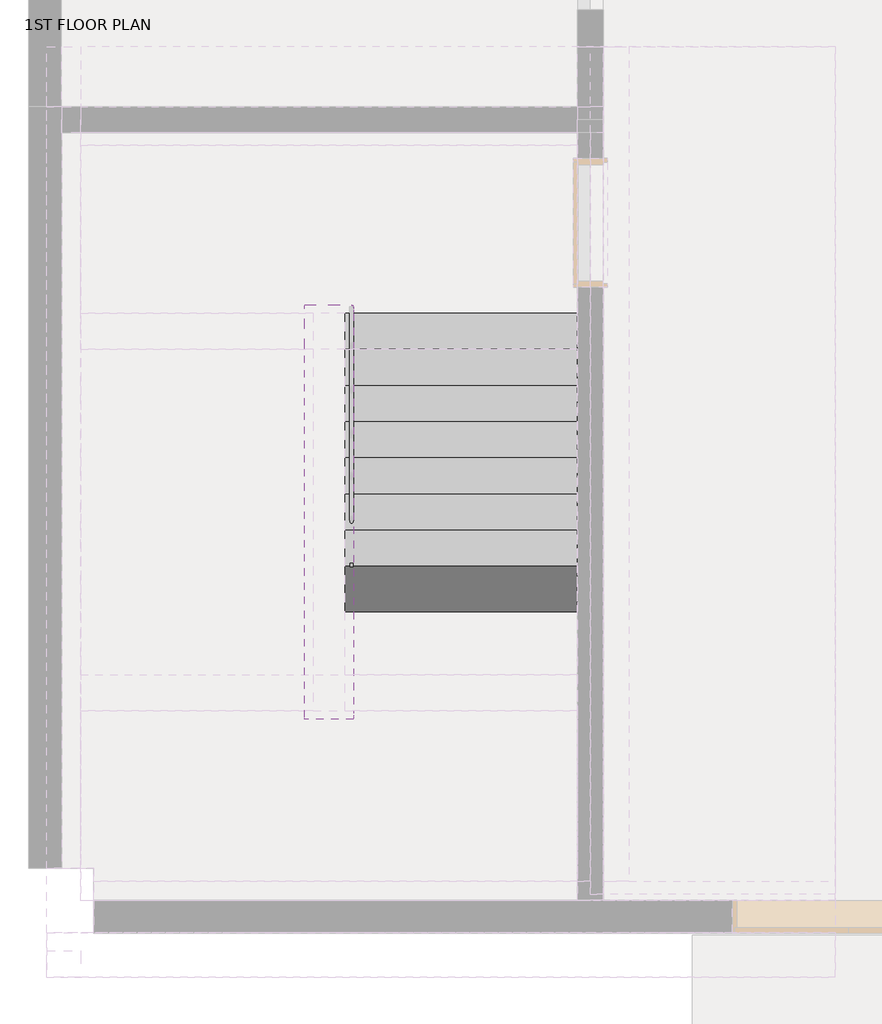
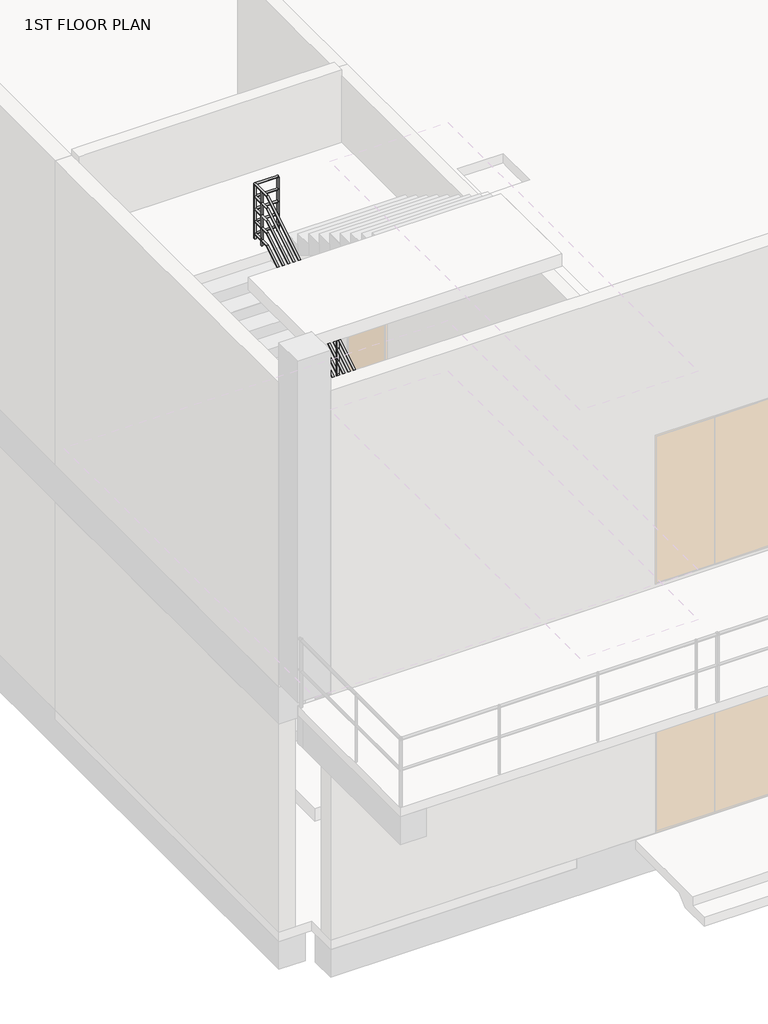
# One storey, part 8 of 9: 1 railing, 1 stair flight.
"""IFC4 building model written with IfcOpenShell, lengths in millimetres."""

from ifc_helpers import new_model, si_unit, frame, origin, place, context, project, spatial, polyline, circle_curve, ellipse_curve, outline, extrude, faceted_brep, element, save
from ifc_brep_helpers import plane_surface, cylinder_surface, advanced_brep

model = new_model("IFC4")

# Units and contexts
model_context = context("Model", 3, world=origin())
ifc_project = project(units=[si_unit("LENGTHUNIT", "METRE", prefix="MILLI")], contexts=[model_context])

# Site, building, storey
site = spatial("IfcSite", under=ifc_project)
building = spatial("IfcBuilding", under=site)
storey = spatial("IfcBuildingStorey", under=building, Name="1ST FLOOR PLAN", Elevation=600.005241)

# Railing
placement = place(None, origin())
element("IfcRailing", 1, ObjectType="900mm 배관", at=placement, inside=storey, context=model_context, shape_type="SolidModel", body=[
    advanced_brep(
    [(2135.0, 25549.5208589, 5485.005241), (2165.0, 25549.5208589, 5485.005241), (2135.0, 25495.2843108, 5485.005241), (2165.0, 25495.2843108, 5485.005241), (2135.0, 22415.2843108, 7375.630241), (2165.0, 22415.2843108, 7375.630241), (2135.0, 22384.5208589, 7375.630241), (2165.0, 22354.5208589, 7375.630241), (1800.0, 22384.5208589, 7375.630241), (1800.0, 22354.5208589, 7375.630241)],
    [
        (0, 1, circle_curve(frame((2150.0, 25549.5208589, 5485.005241), z_axis=(0.0, 1.0, 0.0), x_axis=(1.0, 0.0, 0.0)), 15.0)),
        (1, 0, circle_curve(frame((2150.0, 25549.5208589, 5485.005241), z_axis=(0.0, 1.0, 0.0), x_axis=(1.0, 0.0, 0.0)), 15.0)),
        (0, 2),
        (2, 3, ellipse_curve(frame((2150.0, 25495.2843108, 5485.005241), z_axis=(0.0, 0.9623527489128249, -0.2718035810285242), x_axis=(0.0, 0.2718035810285241, 0.9623527489128249)), 15.5868002, 15.0)),
        (3, 1),
        (3, 2, ellipse_curve(frame((2150.0, 25495.2843108, 5485.005241), z_axis=(0.0, 0.9623527489128249, -0.2718035810285242), x_axis=(0.0, 0.2718035810285241, 0.9623527489128249)), 15.5868002, 15.0)),
        (2, 4),
        (4, 5, ellipse_curve(frame((2150.0, 22415.2843108, 7375.630241), z_axis=(0.0, 0.9623527489128249, -0.27180358102852414), x_axis=(0.0, -0.2718035810285245, -0.9623527489128249)), 15.5868002, 15.0)),
        (5, 3),
        (5, 4, ellipse_curve(frame((2150.0, 22415.2843108, 7375.630241), z_axis=(0.0, 0.9623527489128249, -0.27180358102852414), x_axis=(0.0, -0.2718035810285245, -0.9623527489128249)), 15.5868002, 15.0)),
        (4, 6),
        (6, 7, ellipse_curve(frame((2150.0, 22369.5208589, 7375.630241), z_axis=(0.7071067811865475, 0.7071067811865475, 0.0), x_axis=(-0.7071067811865474, 0.7071067811865476, 0.0)), 21.2132034, 15.0)),
        (7, 5),
        (7, 6, ellipse_curve(frame((2150.0, 22369.5208589, 7375.630241), z_axis=(0.7071067811865475, 0.7071067811865475, 0.0), x_axis=(-0.7071067811865474, 0.7071067811865476, 0.0)), 21.2132034, 15.0)),
        (8, 9, ellipse_curve(frame((1800.0, 22369.5208589, 7375.630241), z_axis=(-0.7071067811865476, 0.0, 0.7071067811865476), x_axis=(0.7071067811865475, 0.0, 0.7071067811865476)), 21.2132034, 15.0)),
        (9, 8, ellipse_curve(frame((1800.0, 22369.5208589, 7375.630241), z_axis=(-0.7071067811865476, 0.0, 0.7071067811865476), x_axis=(0.7071067811865475, 0.0, 0.7071067811865476)), 21.2132034, 15.0)),
        (6, 8),
        (9, 7),
    ],
    [
        plane_surface(frame((2150.0, 25549.5208589, 5500.005241), z_axis=(0.0, 1.0, 0.0), x_axis=(0.0, 0.0, -1.0))),
        cylinder_surface(frame((2150.0, 25549.5208589, 5485.005241), z_axis=(0.0, 1.0, 0.0), x_axis=(1.0, 0.0, 0.0)), 15.0),
        cylinder_surface(frame((2150.0, 25491.6737312, 5487.2215566), z_axis=(0.0, 0.852245626680141, -0.5231418467343), x_axis=(1.0, 0.0, 0.0)), 15.0),
        cylinder_surface(frame((2150.0, 22419.5208589, 7375.630241), z_axis=(0.0, 1.0, 0.0), x_axis=(1.0, 0.0, 0.0)), 15.0),
        plane_surface(frame((1815.0, 22369.5208589, 7390.630241), z_axis=(-0.7071067811865476, 0.0, 0.7071067811865476), x_axis=(0.7071067811865476, 0.0, 0.7071067811865476))),
        cylinder_surface(frame((2150.0, 22369.5208589, 7375.630241), z_axis=(1.0, 0.0, 0.0), x_axis=(0.0, -1.0, 0.0)), 15.0),
    ],
    [
        (0, [[1, 2]]),
        (1, [[-1, 3, 4, 5]]),
        (1, [[-2, -5, 6, -3]]),
        (2, [[-4, 7, 8, 9]]),
        (2, [[-6, -9, 10, -7]]),
        (3, [[-8, 11, 12, 13]]),
        (3, [[-10, -13, 14, -11]]),
        (4, [[15, 16]]),
        (5, [[-12, 17, -16, 18]]),
        (5, [[-14, -18, -15, -17]]),
    ],
),
    advanced_brep(
    [(1800.0, 22384.5208589, 7375.630241), (1800.0, 22354.5208589, 7375.630241), (1800.0, 22384.5208589, 7505.8197466), (1800.0, 22354.5208589, 7522.6056874)],
    [
        (0, 1, ellipse_curve(frame((1800.0, 22369.5208589, 7375.630241), z_axis=(0.7071067811865476, 0.0, -0.7071067811865476), x_axis=(-0.7071067811865476, 0.0, -0.7071067811865474)), 21.2132034, 15.0)),
        (1, 0, ellipse_curve(frame((1800.0, 22369.5208589, 7375.630241), z_axis=(0.7071067811865476, 0.0, -0.7071067811865476), x_axis=(-0.7071067811865476, 0.0, -0.7071067811865474)), 21.2132034, 15.0)),
        (2, 3, ellipse_curve(frame((1800.0, 22369.5208589, 7514.212717), z_axis=(0.0, 0.48829199935371653, 0.8726803099458301), x_axis=(0.0, 0.8726803099458301, -0.4882919993537164)), 17.1884249, 15.0)),
        (3, 2, ellipse_curve(frame((1800.0, 22369.5208589, 7514.212717), z_axis=(0.0, 0.48829199935371653, 0.8726803099458301), x_axis=(0.0, 0.8726803099458301, -0.4882919993537164)), 17.1884249, 15.0)),
        (0, 2),
        (3, 1),
    ],
    [
        plane_surface(frame((1800.0, 22369.5208589, 7375.630241), z_axis=(0.7071067811865476, 0.0, -0.7071067811865476), x_axis=(0.7071067811865476, 0.0, 0.7071067811865476))),
        plane_surface(frame((1800.0, 22369.5208589, 7514.212717), z_axis=(0.0, 0.48829199935371653, 0.8726803099458301), x_axis=(1.0, 0.0, 0.0))),
        cylinder_surface(frame((1800.0, 22369.5208589, 7375.630241), z_axis=(0.0, 0.0, -1.0), x_axis=(0.0, -1.0, 0.0)), 15.0),
    ],
    [
        (0, [[1, 2]]),
        (1, [[3, 4]]),
        (2, [[-1, 5, -4, 6]]),
        (2, [[-2, -6, -3, -5]]),
    ],
),
    advanced_brep(
    [(1815.0, 22369.5208589, 7514.212717), (1785.0, 22369.5208589, 7514.212717), (1815.0, 25223.757407, 9266.255241), (1785.0, 25223.757407, 9266.255241), (1815.0, 25534.5208589, 9266.255241), (1785.0, 25564.5208589, 9266.255241), (2150.0, 25534.5208589, 9266.255241), (2150.0, 25564.5208589, 9266.255241)],
    [
        (0, 1, ellipse_curve(frame((1800.0, 22369.5208589, 7514.212717), z_axis=(0.0, -0.48829199935371653, -0.8726803099458301), x_axis=(0.0, -0.8726803099458302, 0.48829199935371653)), 17.1884249, 15.0)),
        (1, 0, ellipse_curve(frame((1800.0, 22369.5208589, 7514.212717), z_axis=(0.0, -0.48829199935371653, -0.8726803099458301), x_axis=(0.0, -0.8726803099458302, 0.48829199935371653)), 17.1884249, 15.0)),
        (0, 2),
        (2, 3, ellipse_curve(frame((1800.0, 25223.757407, 9266.255241), z_axis=(0.0, -0.9623527489128247, -0.27180358102852437), x_axis=(0.0, 0.2718035810285242, -0.9623527489128249)), 15.5868002, 15.0)),
        (3, 1),
        (3, 2, ellipse_curve(frame((1800.0, 25223.757407, 9266.255241), z_axis=(0.0, -0.9623527489128247, -0.27180358102852437), x_axis=(0.0, 0.2718035810285242, -0.9623527489128249)), 15.5868002, 15.0)),
        (2, 4),
        (4, 5, ellipse_curve(frame((1800.0, 25549.5208589, 9266.255241), z_axis=(-0.7071067811865475, -0.7071067811865475, 0.0), x_axis=(0.7071067811865474, -0.7071067811865476, 0.0)), 21.2132034, 15.0)),
        (5, 3),
        (5, 4, ellipse_curve(frame((1800.0, 25549.5208589, 9266.255241), z_axis=(-0.7071067811865475, -0.7071067811865475, 0.0), x_axis=(0.7071067811865474, -0.7071067811865476, 0.0)), 21.2132034, 15.0)),
        (6, 7, circle_curve(frame((2150.0, 25549.5208589, 9266.255241), z_axis=(1.0, 0.0, 0.0), x_axis=(0.0, 1.0, 0.0)), 15.0)),
        (7, 6, circle_curve(frame((2150.0, 25549.5208589, 9266.255241), z_axis=(1.0, 0.0, 0.0), x_axis=(0.0, 1.0, 0.0)), 15.0)),
        (4, 6),
        (7, 5),
    ],
    [
        plane_surface(frame((1800.0, 22354.5208589, 7522.6056874), z_axis=(0.0, -0.48829199935371653, -0.8726803099458301), x_axis=(1.0, 0.0, 0.0))),
        cylinder_surface(frame((1800.0, 22362.3679866, 7509.822003), z_axis=(0.0, -0.8522456266801408, -0.5231418467343004), x_axis=(-1.0, 0.0, 0.0)), 15.0),
        cylinder_surface(frame((1800.0, 25219.5208589, 9266.255241), z_axis=(0.0, -1.0, 0.0), x_axis=(-1.0, 0.0, 0.0)), 15.0),
        plane_surface(frame((2150.0, 25549.5208589, 9281.255241), z_axis=(1.0, 0.0, 0.0), x_axis=(0.0, 1.0, 0.0))),
        cylinder_surface(frame((1800.0, 25549.5208589, 9266.255241), z_axis=(-1.0, 0.0, 0.0), x_axis=(0.0, 1.0, 0.0)), 15.0),
    ],
    [
        (0, [[1, 2]]),
        (1, [[-1, 3, 4, 5]]),
        (1, [[-2, -5, 6, -3]]),
        (2, [[-4, 7, 8, 9]]),
        (2, [[-6, -9, 10, -7]]),
        (3, [[11, 12]]),
        (4, [[-8, 13, -12, 14]]),
        (4, [[-10, -14, -11, -13]]),
    ],
),
    advanced_brep(
    [(2165.0, 25549.5208589, 5285.005241), (2135.0, 25549.5208589, 5285.005241), (2165.0, 25495.2843108, 5285.005241), (2135.0, 25495.2843108, 5285.005241), (2165.0, 22415.2843108, 7175.630241), (2135.0, 22415.2843108, 7175.630241), (2165.0, 22384.5208589, 7175.630241), (2135.0, 22384.5208589, 7175.630241)],
    [
        (0, 1, circle_curve(frame((2150.0, 25549.5208589, 5285.005241), z_axis=(0.0, 1.0, 0.0), x_axis=(-1.0, 0.0, 0.0)), 15.0)),
        (1, 0, circle_curve(frame((2150.0, 25549.5208589, 5285.005241), z_axis=(0.0, 1.0, 0.0), x_axis=(-1.0, 0.0, 0.0)), 15.0)),
        (0, 2),
        (2, 3, ellipse_curve(frame((2150.0, 25495.2843108, 5285.005241), z_axis=(0.0, 0.9623527489128249, -0.2718035810285242), x_axis=(0.0, 0.2718035810285241, 0.9623527489128249)), 15.5868002, 15.0)),
        (3, 1),
        (3, 2, ellipse_curve(frame((2150.0, 25495.2843108, 5285.005241), z_axis=(0.0, 0.9623527489128249, -0.2718035810285242), x_axis=(0.0, 0.2718035810285241, 0.9623527489128249)), 15.5868002, 15.0)),
        (2, 4),
        (4, 5, ellipse_curve(frame((2150.0, 22415.2843108, 7175.630241), z_axis=(0.0, 0.9623527489128249, -0.27180358102852414), x_axis=(0.0, -0.2718035810285245, -0.9623527489128249)), 15.5868002, 15.0)),
        (5, 3),
        (5, 4, ellipse_curve(frame((2150.0, 22415.2843108, 7175.630241), z_axis=(0.0, 0.9623527489128249, -0.27180358102852414), x_axis=(0.0, -0.2718035810285245, -0.9623527489128249)), 15.5868002, 15.0)),
        (6, 7, circle_curve(frame((2150.0, 22384.5208589, 7175.630241), z_axis=(0.0, -1.0, 0.0), x_axis=(-1.0, 0.0, 0.0)), 15.0)),
        (7, 6, circle_curve(frame((2150.0, 22384.5208589, 7175.630241), z_axis=(0.0, -1.0, 0.0), x_axis=(-1.0, 0.0, 0.0)), 15.0)),
        (4, 6),
        (7, 5),
    ],
    [
        plane_surface(frame((2150.0, 25549.5208589, 5300.005241), z_axis=(0.0, 1.0, 0.0), x_axis=(0.0, 0.0, -1.0))),
        cylinder_surface(frame((2150.0, 25549.5208589, 5285.005241), z_axis=(0.0, 1.0, 0.0), x_axis=(-1.0, 0.0, 0.0)), 15.0),
        cylinder_surface(frame((2150.0, 25491.6737312, 5287.2215566), z_axis=(0.0, 0.852245626680141, -0.5231418467343), x_axis=(-1.0, 0.0, 0.0)), 15.0),
        plane_surface(frame((2150.0, 22384.5208589, 7190.630241), z_axis=(0.0, -1.0, 0.0), x_axis=(0.0, 0.0, -1.0))),
        cylinder_surface(frame((2150.0, 22419.5208589, 7175.630241), z_axis=(0.0, 1.0, 0.0), x_axis=(-1.0, 0.0, 0.0)), 15.0),
    ],
    [
        (0, [[1, 2]]),
        (1, [[-1, 3, 4, 5]]),
        (1, [[-2, -5, 6, -3]]),
        (2, [[-4, 7, 8, 9]]),
        (2, [[-6, -9, 10, -7]]),
        (3, [[11, 12]]),
        (4, [[-8, 13, -12, 14]]),
        (4, [[-10, -14, -11, -13]]),
    ],
),
    advanced_brep(
    [(2165.0, 22354.5208589, 7175.630241), (2165.0, 22384.5208589, 7175.630241), (1815.0, 22354.5208589, 7175.630241), (1815.0, 22384.5208589, 7175.630241)],
    [
        (0, 1, circle_curve(frame((2165.0, 22369.5208589, 7175.630241), z_axis=(1.0, 0.0, 0.0), x_axis=(0.0, 1.0, 0.0)), 15.0)),
        (1, 0, circle_curve(frame((2165.0, 22369.5208589, 7175.630241), z_axis=(1.0, 0.0, 0.0), x_axis=(0.0, 1.0, 0.0)), 15.0)),
        (2, 3, circle_curve(frame((1815.0, 22369.5208589, 7175.630241), z_axis=(-1.0, 0.0, 0.0), x_axis=(0.0, 1.0, 0.0)), 15.0)),
        (3, 2, circle_curve(frame((1815.0, 22369.5208589, 7175.630241), z_axis=(-1.0, 0.0, 0.0), x_axis=(0.0, 1.0, 0.0)), 15.0)),
        (0, 2),
        (3, 1),
    ],
    [
        plane_surface(frame((2165.0, 22369.5208589, 7190.630241), z_axis=(1.0, 0.0, 0.0), x_axis=(0.0, -1.0, 0.0))),
        plane_surface(frame((1815.0, 22369.5208589, 7190.630241), z_axis=(-1.0, 0.0, 0.0), x_axis=(0.0, -1.0, 0.0))),
        cylinder_surface(frame((2165.0, 22369.5208589, 7175.630241), z_axis=(1.0, 0.0, 0.0), x_axis=(0.0, 1.0, 0.0)), 15.0),
    ],
    [
        (0, [[1, 2]]),
        (1, [[3, 4]]),
        (2, [[-1, 5, -4, 6]]),
        (2, [[-2, -6, -3, -5]]),
    ],
),
    advanced_brep(
    [(1785.0, 22354.5208589, 7305.0051277), (1815.0, 22354.5208589, 7305.0051277), (1785.0, 25223.757407, 9066.255241), (1815.0, 25223.757407, 9066.255241), (1785.0, 25534.5208589, 9066.255241), (1815.0, 25534.5208589, 9066.255241)],
    [
        (0, 1, ellipse_curve(frame((1800.0, 22354.5208589, 7305.0051277), z_axis=(0.0, -1.0, 0.0), x_axis=(0.0, 0.0, -1.0)), 17.6005597, 15.0)),
        (1, 0, ellipse_curve(frame((1800.0, 22354.5208589, 7305.0051277), z_axis=(0.0, -1.0, 0.0), x_axis=(0.0, 0.0, -1.0)), 17.6005597, 15.0)),
        (0, 2),
        (2, 3, ellipse_curve(frame((1800.0, 25223.757407, 9066.255241), z_axis=(0.0, -0.9623527489128247, -0.27180358102852437), x_axis=(0.0, 0.2718035810285242, -0.9623527489128249)), 15.5868002, 15.0)),
        (3, 1),
        (3, 2, ellipse_curve(frame((1800.0, 25223.757407, 9066.255241), z_axis=(0.0, -0.9623527489128247, -0.27180358102852437), x_axis=(0.0, 0.2718035810285242, -0.9623527489128249)), 15.5868002, 15.0)),
        (4, 5, circle_curve(frame((1800.0, 25534.5208589, 9066.255241), z_axis=(0.0, 1.0, 0.0), x_axis=(1.0, 0.0, 0.0)), 15.0)),
        (5, 4, circle_curve(frame((1800.0, 25534.5208589, 9066.255241), z_axis=(0.0, 1.0, 0.0), x_axis=(1.0, 0.0, 0.0)), 15.0)),
        (2, 4),
        (5, 3),
    ],
    [
        plane_surface(frame((1800.0, 22354.5208589, 7322.6056874), z_axis=(0.0, -1.0, 0.0), x_axis=(0.0, 0.0, 1.0))),
        cylinder_surface(frame((1800.0, 22362.3679866, 7309.822003), z_axis=(0.0, -0.8522456266801408, -0.5231418467343004), x_axis=(1.0, 0.0, 0.0)), 15.0),
        plane_surface(frame((1800.0, 25534.5208589, 9081.255241), z_axis=(0.0, 1.0, 0.0), x_axis=(0.0, 0.0, 1.0))),
        cylinder_surface(frame((1800.0, 25219.5208589, 9066.255241), z_axis=(0.0, -1.0, 0.0), x_axis=(1.0, 0.0, 0.0)), 15.0),
    ],
    [
        (0, [[1, 2]]),
        (1, [[-1, 3, 4, 5]]),
        (1, [[-2, -5, 6, -3]]),
        (2, [[7, 8]]),
        (3, [[-4, 9, -8, 10]]),
        (3, [[-6, -10, -7, -9]]),
    ],
),
    advanced_brep(
    [(1785.0, 25564.5208589, 9066.255241), (1785.0, 25534.5208589, 9066.255241), (2150.0, 25564.5208589, 9066.255241), (2150.0, 25534.5208589, 9066.255241)],
    [
        (0, 1, circle_curve(frame((1785.0, 25549.5208589, 9066.255241), z_axis=(-1.0, 0.0, 0.0), x_axis=(0.0, -1.0, 0.0)), 15.0)),
        (1, 0, circle_curve(frame((1785.0, 25549.5208589, 9066.255241), z_axis=(-1.0, 0.0, 0.0), x_axis=(0.0, -1.0, 0.0)), 15.0)),
        (2, 3, circle_curve(frame((2150.0, 25549.5208589, 9066.255241), z_axis=(1.0, 0.0, 0.0), x_axis=(0.0, -1.0, 0.0)), 15.0)),
        (3, 2, circle_curve(frame((2150.0, 25549.5208589, 9066.255241), z_axis=(1.0, 0.0, 0.0), x_axis=(0.0, -1.0, 0.0)), 15.0)),
        (0, 2),
        (3, 1),
    ],
    [
        plane_surface(frame((1785.0, 25549.5208589, 9081.255241), z_axis=(-1.0, 0.0, 0.0), x_axis=(0.0, 1.0, 0.0))),
        plane_surface(frame((2150.0, 25549.5208589, 9081.255241), z_axis=(1.0, 0.0, 0.0), x_axis=(0.0, 1.0, 0.0))),
        cylinder_surface(frame((1785.0, 25549.5208589, 9066.255241), z_axis=(-1.0, 0.0, 0.0), x_axis=(0.0, -1.0, 0.0)), 15.0),
    ],
    [
        (0, [[1, 2]]),
        (1, [[3, 4]]),
        (2, [[-1, 5, -4, 6]]),
        (2, [[-2, -6, -3, -5]]),
    ],
),
    advanced_brep(
    [(2165.0, 25549.5208589, 5085.005241), (2135.0, 25549.5208589, 5085.005241), (2165.0, 25495.2843108, 5085.005241), (2135.0, 25495.2843108, 5085.005241), (2165.0, 22415.2843108, 6975.630241), (2135.0, 22415.2843108, 6975.630241), (2165.0, 22384.5208589, 6975.630241), (2135.0, 22384.5208589, 6975.630241)],
    [
        (0, 1, circle_curve(frame((2150.0, 25549.5208589, 5085.005241), z_axis=(0.0, 1.0, 0.0), x_axis=(-1.0, 0.0, 0.0)), 15.0)),
        (1, 0, circle_curve(frame((2150.0, 25549.5208589, 5085.005241), z_axis=(0.0, 1.0, 0.0), x_axis=(-1.0, 0.0, 0.0)), 15.0)),
        (0, 2),
        (2, 3, ellipse_curve(frame((2150.0, 25495.2843108, 5085.005241), z_axis=(0.0, 0.9623527489128249, -0.2718035810285242), x_axis=(0.0, 0.2718035810285241, 0.9623527489128249)), 15.5868002, 15.0)),
        (3, 1),
        (3, 2, ellipse_curve(frame((2150.0, 25495.2843108, 5085.005241), z_axis=(0.0, 0.9623527489128249, -0.2718035810285242), x_axis=(0.0, 0.2718035810285241, 0.9623527489128249)), 15.5868002, 15.0)),
        (2, 4),
        (4, 5, ellipse_curve(frame((2150.0, 22415.2843108, 6975.630241), z_axis=(0.0, 0.9623527489128249, -0.27180358102852414), x_axis=(0.0, -0.2718035810285245, -0.9623527489128249)), 15.5868002, 15.0)),
        (5, 3),
        (5, 4, ellipse_curve(frame((2150.0, 22415.2843108, 6975.630241), z_axis=(0.0, 0.9623527489128249, -0.27180358102852414), x_axis=(0.0, -0.2718035810285245, -0.9623527489128249)), 15.5868002, 15.0)),
        (6, 7, circle_curve(frame((2150.0, 22384.5208589, 6975.630241), z_axis=(0.0, -1.0, 0.0), x_axis=(-1.0, 0.0, 0.0)), 15.0)),
        (7, 6, circle_curve(frame((2150.0, 22384.5208589, 6975.630241), z_axis=(0.0, -1.0, 0.0), x_axis=(-1.0, 0.0, 0.0)), 15.0)),
        (4, 6),
        (7, 5),
    ],
    [
        plane_surface(frame((2150.0, 25549.5208589, 5100.005241), z_axis=(0.0, 1.0, 0.0), x_axis=(0.0, 0.0, -1.0))),
        cylinder_surface(frame((2150.0, 25549.5208589, 5085.005241), z_axis=(0.0, 1.0, 0.0), x_axis=(-1.0, 0.0, 0.0)), 15.0),
        cylinder_surface(frame((2150.0, 25491.6737312, 5087.2215566), z_axis=(0.0, 0.852245626680141, -0.5231418467343), x_axis=(-1.0, 0.0, 0.0)), 15.0),
        plane_surface(frame((2150.0, 22384.5208589, 6990.630241), z_axis=(0.0, -1.0, 0.0), x_axis=(0.0, 0.0, -1.0))),
        cylinder_surface(frame((2150.0, 22419.5208589, 6975.630241), z_axis=(0.0, 1.0, 0.0), x_axis=(-1.0, 0.0, 0.0)), 15.0),
    ],
    [
        (0, [[1, 2]]),
        (1, [[-1, 3, 4, 5]]),
        (1, [[-2, -5, 6, -3]]),
        (2, [[-4, 7, 8, 9]]),
        (2, [[-6, -9, 10, -7]]),
        (3, [[11, 12]]),
        (4, [[-8, 13, -12, 14]]),
        (4, [[-10, -14, -11, -13]]),
    ],
),
    advanced_brep(
    [(2165.0, 22354.5208589, 6975.630241), (2165.0, 22384.5208589, 6975.630241), (1815.0, 22354.5208589, 6975.630241), (1815.0, 22384.5208589, 6975.630241)],
    [
        (0, 1, circle_curve(frame((2165.0, 22369.5208589, 6975.630241), z_axis=(1.0, 0.0, 0.0), x_axis=(0.0, 1.0, 0.0)), 15.0)),
        (1, 0, circle_curve(frame((2165.0, 22369.5208589, 6975.630241), z_axis=(1.0, 0.0, 0.0), x_axis=(0.0, 1.0, 0.0)), 15.0)),
        (2, 3, circle_curve(frame((1815.0, 22369.5208589, 6975.630241), z_axis=(-1.0, 0.0, 0.0), x_axis=(0.0, 1.0, 0.0)), 15.0)),
        (3, 2, circle_curve(frame((1815.0, 22369.5208589, 6975.630241), z_axis=(-1.0, 0.0, 0.0), x_axis=(0.0, 1.0, 0.0)), 15.0)),
        (0, 2),
        (3, 1),
    ],
    [
        plane_surface(frame((2165.0, 22369.5208589, 6990.630241), z_axis=(1.0, 0.0, 0.0), x_axis=(0.0, -1.0, 0.0))),
        plane_surface(frame((1815.0, 22369.5208589, 6990.630241), z_axis=(-1.0, 0.0, 0.0), x_axis=(0.0, -1.0, 0.0))),
        cylinder_surface(frame((2165.0, 22369.5208589, 6975.630241), z_axis=(1.0, 0.0, 0.0), x_axis=(0.0, 1.0, 0.0)), 15.0),
    ],
    [
        (0, [[1, 2]]),
        (1, [[3, 4]]),
        (2, [[-1, 5, -4, 6]]),
        (2, [[-2, -6, -3, -5]]),
    ],
),
    advanced_brep(
    [(1785.0, 22354.5208589, 7105.0051277), (1815.0, 22354.5208589, 7105.0051277), (1785.0, 25223.757407, 8866.255241), (1815.0, 25223.757407, 8866.255241), (1785.0, 25534.5208589, 8866.255241), (1815.0, 25534.5208589, 8866.255241)],
    [
        (0, 1, ellipse_curve(frame((1800.0, 22354.5208589, 7105.0051277), z_axis=(0.0, -1.0, 0.0), x_axis=(0.0, 0.0, -1.0)), 17.6005597, 15.0)),
        (1, 0, ellipse_curve(frame((1800.0, 22354.5208589, 7105.0051277), z_axis=(0.0, -1.0, 0.0), x_axis=(0.0, 0.0, -1.0)), 17.6005597, 15.0)),
        (0, 2),
        (2, 3, ellipse_curve(frame((1800.0, 25223.757407, 8866.255241), z_axis=(0.0, -0.9623527489128247, -0.27180358102852437), x_axis=(0.0, 0.2718035810285242, -0.9623527489128249)), 15.5868002, 15.0)),
        (3, 1),
        (3, 2, ellipse_curve(frame((1800.0, 25223.757407, 8866.255241), z_axis=(0.0, -0.9623527489128247, -0.27180358102852437), x_axis=(0.0, 0.2718035810285242, -0.9623527489128249)), 15.5868002, 15.0)),
        (4, 5, circle_curve(frame((1800.0, 25534.5208589, 8866.255241), z_axis=(0.0, 1.0, 0.0), x_axis=(1.0, 0.0, 0.0)), 15.0)),
        (5, 4, circle_curve(frame((1800.0, 25534.5208589, 8866.255241), z_axis=(0.0, 1.0, 0.0), x_axis=(1.0, 0.0, 0.0)), 15.0)),
        (2, 4),
        (5, 3),
    ],
    [
        plane_surface(frame((1800.0, 22354.5208589, 7122.6056874), z_axis=(0.0, -1.0, 0.0), x_axis=(0.0, 0.0, 1.0))),
        cylinder_surface(frame((1800.0, 22362.3679866, 7109.822003), z_axis=(0.0, -0.8522456266801408, -0.5231418467343004), x_axis=(1.0, 0.0, 0.0)), 15.0),
        plane_surface(frame((1800.0, 25534.5208589, 8881.255241), z_axis=(0.0, 1.0, 0.0), x_axis=(0.0, 0.0, 1.0))),
        cylinder_surface(frame((1800.0, 25219.5208589, 8866.255241), z_axis=(0.0, -1.0, 0.0), x_axis=(1.0, 0.0, 0.0)), 15.0),
    ],
    [
        (0, [[1, 2]]),
        (1, [[-1, 3, 4, 5]]),
        (1, [[-2, -5, 6, -3]]),
        (2, [[7, 8]]),
        (3, [[-4, 9, -8, 10]]),
        (3, [[-6, -10, -7, -9]]),
    ],
),
    advanced_brep(
    [(1785.0, 25564.5208589, 8866.255241), (1785.0, 25534.5208589, 8866.255241), (2150.0, 25564.5208589, 8866.255241), (2150.0, 25534.5208589, 8866.255241)],
    [
        (0, 1, circle_curve(frame((1785.0, 25549.5208589, 8866.255241), z_axis=(-1.0, 0.0, 0.0), x_axis=(0.0, -1.0, 0.0)), 15.0)),
        (1, 0, circle_curve(frame((1785.0, 25549.5208589, 8866.255241), z_axis=(-1.0, 0.0, 0.0), x_axis=(0.0, -1.0, 0.0)), 15.0)),
        (2, 3, circle_curve(frame((2150.0, 25549.5208589, 8866.255241), z_axis=(1.0, 0.0, 0.0), x_axis=(0.0, -1.0, 0.0)), 15.0)),
        (3, 2, circle_curve(frame((2150.0, 25549.5208589, 8866.255241), z_axis=(1.0, 0.0, 0.0), x_axis=(0.0, -1.0, 0.0)), 15.0)),
        (0, 2),
        (3, 1),
    ],
    [
        plane_surface(frame((1785.0, 25549.5208589, 8881.255241), z_axis=(-1.0, 0.0, 0.0), x_axis=(0.0, 1.0, 0.0))),
        plane_surface(frame((2150.0, 25549.5208589, 8881.255241), z_axis=(1.0, 0.0, 0.0), x_axis=(0.0, 1.0, 0.0))),
        cylinder_surface(frame((1785.0, 25549.5208589, 8866.255241), z_axis=(-1.0, 0.0, 0.0), x_axis=(0.0, -1.0, 0.0)), 15.0),
    ],
    [
        (0, [[1, 2]]),
        (1, [[3, 4]]),
        (2, [[-1, 5, -4, 6]]),
        (2, [[-2, -6, -3, -5]]),
    ],
),
    advanced_brep(
    [(2165.0, 25549.5208589, 4885.005241), (2135.0, 25549.5208589, 4885.005241), (2165.0, 25495.2843108, 4885.005241), (2135.0, 25495.2843108, 4885.005241), (2165.0, 22415.2843108, 6775.630241), (2135.0, 22415.2843108, 6775.630241), (2165.0, 22384.5208589, 6775.630241), (2135.0, 22384.5208589, 6775.630241)],
    [
        (0, 1, circle_curve(frame((2150.0, 25549.5208589, 4885.005241), z_axis=(0.0, 1.0, 0.0), x_axis=(-1.0, 0.0, 0.0)), 15.0)),
        (1, 0, circle_curve(frame((2150.0, 25549.5208589, 4885.005241), z_axis=(0.0, 1.0, 0.0), x_axis=(-1.0, 0.0, 0.0)), 15.0)),
        (0, 2),
        (2, 3, ellipse_curve(frame((2150.0, 25495.2843108, 4885.005241), z_axis=(0.0, 0.9623527489128249, -0.2718035810285242), x_axis=(0.0, 0.2718035810285241, 0.9623527489128249)), 15.5868002, 15.0)),
        (3, 1),
        (3, 2, ellipse_curve(frame((2150.0, 25495.2843108, 4885.005241), z_axis=(0.0, 0.9623527489128249, -0.2718035810285242), x_axis=(0.0, 0.2718035810285241, 0.9623527489128249)), 15.5868002, 15.0)),
        (2, 4),
        (4, 5, ellipse_curve(frame((2150.0, 22415.2843108, 6775.630241), z_axis=(0.0, 0.9623527489128249, -0.27180358102852414), x_axis=(0.0, -0.2718035810285245, -0.9623527489128249)), 15.5868002, 15.0)),
        (5, 3),
        (5, 4, ellipse_curve(frame((2150.0, 22415.2843108, 6775.630241), z_axis=(0.0, 0.9623527489128249, -0.27180358102852414), x_axis=(0.0, -0.2718035810285245, -0.9623527489128249)), 15.5868002, 15.0)),
        (6, 7, circle_curve(frame((2150.0, 22384.5208589, 6775.630241), z_axis=(0.0, -1.0, 0.0), x_axis=(-1.0, 0.0, 0.0)), 15.0)),
        (7, 6, circle_curve(frame((2150.0, 22384.5208589, 6775.630241), z_axis=(0.0, -1.0, 0.0), x_axis=(-1.0, 0.0, 0.0)), 15.0)),
        (4, 6),
        (7, 5),
    ],
    [
        plane_surface(frame((2150.0, 25549.5208589, 4900.005241), z_axis=(0.0, 1.0, 0.0), x_axis=(0.0, 0.0, -1.0))),
        cylinder_surface(frame((2150.0, 25549.5208589, 4885.005241), z_axis=(0.0, 1.0, 0.0), x_axis=(-1.0, 0.0, 0.0)), 15.0),
        cylinder_surface(frame((2150.0, 25491.6737312, 4887.2215566), z_axis=(0.0, 0.852245626680141, -0.5231418467343), x_axis=(-1.0, 0.0, 0.0)), 15.0),
        plane_surface(frame((2150.0, 22384.5208589, 6790.630241), z_axis=(0.0, -1.0, 0.0), x_axis=(0.0, 0.0, -1.0))),
        cylinder_surface(frame((2150.0, 22419.5208589, 6775.630241), z_axis=(0.0, 1.0, 0.0), x_axis=(-1.0, 0.0, 0.0)), 15.0),
    ],
    [
        (0, [[1, 2]]),
        (1, [[-1, 3, 4, 5]]),
        (1, [[-2, -5, 6, -3]]),
        (2, [[-4, 7, 8, 9]]),
        (2, [[-6, -9, 10, -7]]),
        (3, [[11, 12]]),
        (4, [[-8, 13, -12, 14]]),
        (4, [[-10, -14, -11, -13]]),
    ],
),
    advanced_brep(
    [(2165.0, 22354.5208589, 6775.630241), (2165.0, 22384.5208589, 6775.630241), (1815.0, 22354.5208589, 6775.630241), (1815.0, 22384.5208589, 6775.630241)],
    [
        (0, 1, circle_curve(frame((2165.0, 22369.5208589, 6775.630241), z_axis=(1.0, 0.0, 0.0), x_axis=(0.0, 1.0, 0.0)), 15.0)),
        (1, 0, circle_curve(frame((2165.0, 22369.5208589, 6775.630241), z_axis=(1.0, 0.0, 0.0), x_axis=(0.0, 1.0, 0.0)), 15.0)),
        (2, 3, circle_curve(frame((1815.0, 22369.5208589, 6775.630241), z_axis=(-1.0, 0.0, 0.0), x_axis=(0.0, 1.0, 0.0)), 15.0)),
        (3, 2, circle_curve(frame((1815.0, 22369.5208589, 6775.630241), z_axis=(-1.0, 0.0, 0.0), x_axis=(0.0, 1.0, 0.0)), 15.0)),
        (0, 2),
        (3, 1),
    ],
    [
        plane_surface(frame((2165.0, 22369.5208589, 6790.630241), z_axis=(1.0, 0.0, 0.0), x_axis=(0.0, -1.0, 0.0))),
        plane_surface(frame((1815.0, 22369.5208589, 6790.630241), z_axis=(-1.0, 0.0, 0.0), x_axis=(0.0, -1.0, 0.0))),
        cylinder_surface(frame((2165.0, 22369.5208589, 6775.630241), z_axis=(1.0, 0.0, 0.0), x_axis=(0.0, 1.0, 0.0)), 15.0),
    ],
    [
        (0, [[1, 2]]),
        (1, [[3, 4]]),
        (2, [[-1, 5, -4, 6]]),
        (2, [[-2, -6, -3, -5]]),
    ],
),
    advanced_brep(
    [(1785.0, 22354.5208589, 6905.0051277), (1815.0, 22354.5208589, 6905.0051277), (1785.0, 25223.757407, 8666.255241), (1815.0, 25223.757407, 8666.255241), (1785.0, 25534.5208589, 8666.255241), (1815.0, 25534.5208589, 8666.255241)],
    [
        (0, 1, ellipse_curve(frame((1800.0, 22354.5208589, 6905.0051277), z_axis=(0.0, -1.0, 0.0), x_axis=(0.0, 0.0, -1.0)), 17.6005597, 15.0)),
        (1, 0, ellipse_curve(frame((1800.0, 22354.5208589, 6905.0051277), z_axis=(0.0, -1.0, 0.0), x_axis=(0.0, 0.0, -1.0)), 17.6005597, 15.0)),
        (0, 2),
        (2, 3, ellipse_curve(frame((1800.0, 25223.757407, 8666.255241), z_axis=(0.0, -0.9623527489128247, -0.27180358102852437), x_axis=(0.0, 0.2718035810285242, -0.9623527489128249)), 15.5868002, 15.0)),
        (3, 1),
        (3, 2, ellipse_curve(frame((1800.0, 25223.757407, 8666.255241), z_axis=(0.0, -0.9623527489128247, -0.27180358102852437), x_axis=(0.0, 0.2718035810285242, -0.9623527489128249)), 15.5868002, 15.0)),
        (4, 5, circle_curve(frame((1800.0, 25534.5208589, 8666.255241), z_axis=(0.0, 1.0, 0.0), x_axis=(1.0, 0.0, 0.0)), 15.0)),
        (5, 4, circle_curve(frame((1800.0, 25534.5208589, 8666.255241), z_axis=(0.0, 1.0, 0.0), x_axis=(1.0, 0.0, 0.0)), 15.0)),
        (2, 4),
        (5, 3),
    ],
    [
        plane_surface(frame((1800.0, 22354.5208589, 6922.6056874), z_axis=(0.0, -1.0, 0.0), x_axis=(0.0, 0.0, 1.0))),
        cylinder_surface(frame((1800.0, 22362.3679866, 6909.822003), z_axis=(0.0, -0.8522456266801408, -0.5231418467343004), x_axis=(1.0, 0.0, 0.0)), 15.0),
        plane_surface(frame((1800.0, 25534.5208589, 8681.255241), z_axis=(0.0, 1.0, 0.0), x_axis=(0.0, 0.0, 1.0))),
        cylinder_surface(frame((1800.0, 25219.5208589, 8666.255241), z_axis=(0.0, -1.0, 0.0), x_axis=(1.0, 0.0, 0.0)), 15.0),
    ],
    [
        (0, [[1, 2]]),
        (1, [[-1, 3, 4, 5]]),
        (1, [[-2, -5, 6, -3]]),
        (2, [[7, 8]]),
        (3, [[-4, 9, -8, 10]]),
        (3, [[-6, -10, -7, -9]]),
    ],
),
    advanced_brep(
    [(1785.0, 25564.5208589, 8666.255241), (1785.0, 25534.5208589, 8666.255241), (2150.0, 25564.5208589, 8666.255241), (2150.0, 25534.5208589, 8666.255241)],
    [
        (0, 1, circle_curve(frame((1785.0, 25549.5208589, 8666.255241), z_axis=(-1.0, 0.0, 0.0), x_axis=(0.0, -1.0, 0.0)), 15.0)),
        (1, 0, circle_curve(frame((1785.0, 25549.5208589, 8666.255241), z_axis=(-1.0, 0.0, 0.0), x_axis=(0.0, -1.0, 0.0)), 15.0)),
        (2, 3, circle_curve(frame((2150.0, 25549.5208589, 8666.255241), z_axis=(1.0, 0.0, 0.0), x_axis=(0.0, -1.0, 0.0)), 15.0)),
        (3, 2, circle_curve(frame((2150.0, 25549.5208589, 8666.255241), z_axis=(1.0, 0.0, 0.0), x_axis=(0.0, -1.0, 0.0)), 15.0)),
        (0, 2),
        (3, 1),
    ],
    [
        plane_surface(frame((1785.0, 25549.5208589, 8681.255241), z_axis=(-1.0, 0.0, 0.0), x_axis=(0.0, 1.0, 0.0))),
        plane_surface(frame((2150.0, 25549.5208589, 8681.255241), z_axis=(1.0, 0.0, 0.0), x_axis=(0.0, 1.0, 0.0))),
        cylinder_surface(frame((1785.0, 25549.5208589, 8666.255241), z_axis=(-1.0, 0.0, 0.0), x_axis=(0.0, -1.0, 0.0)), 15.0),
    ],
    [
        (0, [[1, 2]]),
        (1, [[3, 4]]),
        (2, [[-1, 5, -4, 6]]),
        (2, [[-2, -6, -3, -5]]),
    ],
),
    advanced_brep(
    [(2165.0, 25549.5208589, 4685.005241), (2135.0, 25549.5208589, 4685.005241), (2165.0, 25495.2843108, 4685.005241), (2135.0, 25495.2843108, 4685.005241), (2165.0, 22415.2843108, 6575.630241), (2135.0, 22415.2843108, 6575.630241), (2165.0, 22384.5208589, 6575.630241), (2135.0, 22384.5208589, 6575.630241)],
    [
        (0, 1, circle_curve(frame((2150.0, 25549.5208589, 4685.005241), z_axis=(0.0, 1.0, 0.0), x_axis=(-1.0, 0.0, 0.0)), 15.0)),
        (1, 0, circle_curve(frame((2150.0, 25549.5208589, 4685.005241), z_axis=(0.0, 1.0, 0.0), x_axis=(-1.0, 0.0, 0.0)), 15.0)),
        (0, 2),
        (2, 3, ellipse_curve(frame((2150.0, 25495.2843108, 4685.005241), z_axis=(0.0, 0.9623527489128249, -0.2718035810285242), x_axis=(0.0, 0.2718035810285241, 0.9623527489128249)), 15.5868002, 15.0)),
        (3, 1),
        (3, 2, ellipse_curve(frame((2150.0, 25495.2843108, 4685.005241), z_axis=(0.0, 0.9623527489128249, -0.2718035810285242), x_axis=(0.0, 0.2718035810285241, 0.9623527489128249)), 15.5868002, 15.0)),
        (2, 4),
        (4, 5, ellipse_curve(frame((2150.0, 22415.2843108, 6575.630241), z_axis=(0.0, 0.9623527489128249, -0.27180358102852414), x_axis=(0.0, -0.2718035810285245, -0.9623527489128249)), 15.5868002, 15.0)),
        (5, 3),
        (5, 4, ellipse_curve(frame((2150.0, 22415.2843108, 6575.630241), z_axis=(0.0, 0.9623527489128249, -0.27180358102852414), x_axis=(0.0, -0.2718035810285245, -0.9623527489128249)), 15.5868002, 15.0)),
        (6, 7, circle_curve(frame((2150.0, 22384.5208589, 6575.630241), z_axis=(0.0, -1.0, 0.0), x_axis=(-1.0, 0.0, 0.0)), 15.0)),
        (7, 6, circle_curve(frame((2150.0, 22384.5208589, 6575.630241), z_axis=(0.0, -1.0, 0.0), x_axis=(-1.0, 0.0, 0.0)), 15.0)),
        (4, 6),
        (7, 5),
    ],
    [
        plane_surface(frame((2150.0, 25549.5208589, 4700.005241), z_axis=(0.0, 1.0, 0.0), x_axis=(0.0, 0.0, -1.0))),
        cylinder_surface(frame((2150.0, 25549.5208589, 4685.005241), z_axis=(0.0, 1.0, 0.0), x_axis=(-1.0, 0.0, 0.0)), 15.0),
        cylinder_surface(frame((2150.0, 25491.6737312, 4687.2215566), z_axis=(0.0, 0.852245626680141, -0.5231418467343), x_axis=(-1.0, 0.0, 0.0)), 15.0),
        plane_surface(frame((2150.0, 22384.5208589, 6590.630241), z_axis=(0.0, -1.0, 0.0), x_axis=(0.0, 0.0, -1.0))),
        cylinder_surface(frame((2150.0, 22419.5208589, 6575.630241), z_axis=(0.0, 1.0, 0.0), x_axis=(-1.0, 0.0, 0.0)), 15.0),
    ],
    [
        (0, [[1, 2]]),
        (1, [[-1, 3, 4, 5]]),
        (1, [[-2, -5, 6, -3]]),
        (2, [[-4, 7, 8, 9]]),
        (2, [[-6, -9, 10, -7]]),
        (3, [[11, 12]]),
        (4, [[-8, 13, -12, 14]]),
        (4, [[-10, -14, -11, -13]]),
    ],
),
    advanced_brep(
    [(2165.0, 22354.5208589, 6575.630241), (2165.0, 22384.5208589, 6575.630241), (1815.0, 22354.5208589, 6575.630241), (1815.0, 22384.5208589, 6575.630241)],
    [
        (0, 1, circle_curve(frame((2165.0, 22369.5208589, 6575.630241), z_axis=(1.0, 0.0, 0.0), x_axis=(0.0, 1.0, 0.0)), 15.0)),
        (1, 0, circle_curve(frame((2165.0, 22369.5208589, 6575.630241), z_axis=(1.0, 0.0, 0.0), x_axis=(0.0, 1.0, 0.0)), 15.0)),
        (2, 3, circle_curve(frame((1815.0, 22369.5208589, 6575.630241), z_axis=(-1.0, 0.0, 0.0), x_axis=(0.0, 1.0, 0.0)), 15.0)),
        (3, 2, circle_curve(frame((1815.0, 22369.5208589, 6575.630241), z_axis=(-1.0, 0.0, 0.0), x_axis=(0.0, 1.0, 0.0)), 15.0)),
        (0, 2),
        (3, 1),
    ],
    [
        plane_surface(frame((2165.0, 22369.5208589, 6590.630241), z_axis=(1.0, 0.0, 0.0), x_axis=(0.0, -1.0, 0.0))),
        plane_surface(frame((1815.0, 22369.5208589, 6590.630241), z_axis=(-1.0, 0.0, 0.0), x_axis=(0.0, -1.0, 0.0))),
        cylinder_surface(frame((2165.0, 22369.5208589, 6575.630241), z_axis=(1.0, 0.0, 0.0), x_axis=(0.0, 1.0, 0.0)), 15.0),
    ],
    [
        (0, [[1, 2]]),
        (1, [[3, 4]]),
        (2, [[-1, 5, -4, 6]]),
        (2, [[-2, -6, -3, -5]]),
    ],
),
    advanced_brep(
    [(1785.0, 22354.5208589, 6705.0051277), (1815.0, 22354.5208589, 6705.0051277), (1785.0, 25223.757407, 8466.255241), (1815.0, 25223.757407, 8466.255241), (1785.0, 25534.5208589, 8466.255241), (1815.0, 25534.5208589, 8466.255241)],
    [
        (0, 1, ellipse_curve(frame((1800.0, 22354.5208589, 6705.0051277), z_axis=(0.0, -1.0, 0.0), x_axis=(0.0, 0.0, -1.0)), 17.6005597, 15.0)),
        (1, 0, ellipse_curve(frame((1800.0, 22354.5208589, 6705.0051277), z_axis=(0.0, -1.0, 0.0), x_axis=(0.0, 0.0, -1.0)), 17.6005597, 15.0)),
        (0, 2),
        (2, 3, ellipse_curve(frame((1800.0, 25223.757407, 8466.255241), z_axis=(0.0, -0.9623527489128247, -0.27180358102852437), x_axis=(0.0, 0.2718035810285242, -0.9623527489128249)), 15.5868002, 15.0)),
        (3, 1),
        (3, 2, ellipse_curve(frame((1800.0, 25223.757407, 8466.255241), z_axis=(0.0, -0.9623527489128247, -0.27180358102852437), x_axis=(0.0, 0.2718035810285242, -0.9623527489128249)), 15.5868002, 15.0)),
        (4, 5, circle_curve(frame((1800.0, 25534.5208589, 8466.255241), z_axis=(0.0, 1.0, 0.0), x_axis=(1.0, 0.0, 0.0)), 15.0)),
        (5, 4, circle_curve(frame((1800.0, 25534.5208589, 8466.255241), z_axis=(0.0, 1.0, 0.0), x_axis=(1.0, 0.0, 0.0)), 15.0)),
        (2, 4),
        (5, 3),
    ],
    [
        plane_surface(frame((1800.0, 22354.5208589, 6722.6056874), z_axis=(0.0, -1.0, 0.0), x_axis=(0.0, 0.0, 1.0))),
        cylinder_surface(frame((1800.0, 22362.3679866, 6709.822003), z_axis=(0.0, -0.8522456266801408, -0.5231418467343004), x_axis=(1.0, 0.0, 0.0)), 15.0),
        plane_surface(frame((1800.0, 25534.5208589, 8481.255241), z_axis=(0.0, 1.0, 0.0), x_axis=(0.0, 0.0, 1.0))),
        cylinder_surface(frame((1800.0, 25219.5208589, 8466.255241), z_axis=(0.0, -1.0, 0.0), x_axis=(1.0, 0.0, 0.0)), 15.0),
    ],
    [
        (0, [[1, 2]]),
        (1, [[-1, 3, 4, 5]]),
        (1, [[-2, -5, 6, -3]]),
        (2, [[7, 8]]),
        (3, [[-4, 9, -8, 10]]),
        (3, [[-6, -10, -7, -9]]),
    ],
),
    advanced_brep(
    [(1785.0, 25564.5208589, 8466.255241), (1785.0, 25534.5208589, 8466.255241), (2150.0, 25564.5208589, 8466.255241), (2150.0, 25534.5208589, 8466.255241)],
    [
        (0, 1, circle_curve(frame((1785.0, 25549.5208589, 8466.255241), z_axis=(-1.0, 0.0, 0.0), x_axis=(0.0, -1.0, 0.0)), 15.0)),
        (1, 0, circle_curve(frame((1785.0, 25549.5208589, 8466.255241), z_axis=(-1.0, 0.0, 0.0), x_axis=(0.0, -1.0, 0.0)), 15.0)),
        (2, 3, circle_curve(frame((2150.0, 25549.5208589, 8466.255241), z_axis=(1.0, 0.0, 0.0), x_axis=(0.0, -1.0, 0.0)), 15.0)),
        (3, 2, circle_curve(frame((2150.0, 25549.5208589, 8466.255241), z_axis=(1.0, 0.0, 0.0), x_axis=(0.0, -1.0, 0.0)), 15.0)),
        (0, 2),
        (3, 1),
    ],
    [
        plane_surface(frame((1785.0, 25549.5208589, 8481.255241), z_axis=(-1.0, 0.0, 0.0), x_axis=(0.0, 1.0, 0.0))),
        plane_surface(frame((2150.0, 25549.5208589, 8481.255241), z_axis=(1.0, 0.0, 0.0), x_axis=(0.0, 1.0, 0.0))),
        cylinder_surface(frame((1785.0, 25549.5208589, 8466.255241), z_axis=(-1.0, 0.0, 0.0), x_axis=(0.0, -1.0, 0.0)), 15.0),
    ],
    [
        (0, [[1, 2]]),
        (1, [[3, 4]]),
        (2, [[-1, 5, -4, 6]]),
        (2, [[-2, -6, -3, -5]]),
    ],
),
    extrude(outline(polyline([(1812.5, 25357.0208589), (1787.5, 25357.0208589), (1787.5, 25382.0208589), (1812.5, 25382.0208589), (1812.5, 25357.0208589)])), frame((0.0, 0.0, 8381.255241), z_axis=(0.0, 0.0, 1.0), x_axis=(1.0, 0.0, 0.0)), (0.0, 0.0, 1.0), 870.0),
    extrude(outline(polyline([(24357.0208589, 8716.6177377), (24382.0208589, 8731.9637199), (24382.0208589, 7693.755241), (24357.0208589, 7693.755241), (24357.0208589, 8716.6177377)])), frame((1787.5, 0.0, 0.0), z_axis=(1.0, 0.0, 0.0), x_axis=(0.0, 1.0, 0.0)), (0.0, 0.0, 1.0), 25.0),
    extrude(outline(polyline([(23357.0208589, 8102.778452), (23382.0208589, 8118.1244341), (23382.0208589, 7178.130241), (23357.0208589, 7178.130241), (23357.0208589, 8102.778452)])), frame((1787.5, 0.0, 0.0), z_axis=(1.0, 0.0, 0.0), x_axis=(0.0, 1.0, 0.0)), (0.0, 0.0, 1.0), 25.0),
    extrude(outline(polyline([(22537.0208589, 7283.3030056), (22562.0208589, 7267.9570234), (22562.0208589, 6318.755241), (22537.0208589, 6318.755241), (22537.0208589, 7283.3030056)])), frame((2137.5, 0.0, 0.0), z_axis=(1.0, 0.0, 0.0), x_axis=(0.0, 1.0, 0.0)), (0.0, 0.0, 1.0), 25.0),
    extrude(outline(polyline([(23537.0208589, 6669.4637199), (23562.0208589, 6654.1177377), (23562.0208589, 5631.255241), (23537.0208589, 5631.255241), (23537.0208589, 6669.4637199)])), frame((2137.5, 0.0, 0.0), z_axis=(1.0, 0.0, 0.0), x_axis=(0.0, 1.0, 0.0)), (0.0, 0.0, 1.0), 25.0),
    extrude(outline(polyline([(24537.0208589, 6055.6244341), (24562.0208589, 6040.278452), (24562.0208589, 5115.630241), (24537.0208589, 5115.630241), (24537.0208589, 6055.6244341)])), frame((2137.5, 0.0, 0.0), z_axis=(1.0, 0.0, 0.0), x_axis=(0.0, 1.0, 0.0)), (0.0, 0.0, 1.0), 25.0),
    extrude(outline(polyline([(2137.5, 25537.0208589), (2137.5, 25562.0208589), (2162.5, 25562.0208589), (2162.5, 25537.0208589), (2137.5, 25537.0208589)])), frame((0.0, 0.0, 8381.255241), z_axis=(0.0, 0.0, 1.0), x_axis=(1.0, 0.0, 0.0)), (0.0, 0.0, 1.0), 870.0),
    extrude(outline(polyline([(1812.5, 25537.0208589), (1787.5, 25537.0208589), (1787.5, 25562.0208589), (1812.5, 25562.0208589), (1812.5, 25537.0208589)])), frame((0.0, 0.0, 8381.255241), z_axis=(0.0, 0.0, 1.0), x_axis=(1.0, 0.0, 0.0)), (0.0, 0.0, 1.0), 870.0),
    extrude(outline(polyline([(1812.5, 22382.0208589), (1812.5, 22357.0208589), (1787.5, 22357.0208589), (1787.5, 22382.0208589), (1812.5, 22382.0208589)])), frame((0.0, 0.0, 6490.630241), z_axis=(0.0, 0.0, 1.0), x_axis=(1.0, 0.0, 0.0)), (0.0, 0.0, 1.0), 870.0),
    extrude(outline(polyline([(2137.5, 22382.0208589), (2162.5, 22382.0208589), (2162.5, 22357.0208589), (2137.5, 22357.0208589), (2137.5, 22382.0208589)])), frame((0.0, 0.0, 6490.630241), z_axis=(0.0, 0.0, 1.0), x_axis=(1.0, 0.0, 0.0)), (0.0, 0.0, 1.0), 870.0),
])

# Stair flight
element("IfcStairFlight", 2, ObjectType="1mm 디딤판", at=placement, inside=storey, context=model_context, shape_type="SolidModel", body=[
    faceted_brep([(3900.0, 25219.5208589, 765.8781576), (3900.0, 25499.5208589, 765.8781576), (2100.0, 25499.5208589, 765.8781576), (2100.0, 25219.5208589, 765.8781576), (3900.0, 25219.5208589, 600.005241), (3900.0, 25499.5208589, 600.005241), (2100.0, 25499.5208589, 600.005241), (2100.0, 25219.5208589, 600.005241), (3900.0, 24939.5208589, 932.5448243), (3900.0, 25219.5208589, 932.5448243), (2100.0, 25219.5208589, 932.5448243), (2100.0, 24939.5208589, 932.5448243), (3900.0, 24939.5208589, 757.9826899), (3900.0, 25204.9229731, 600.005241), (2100.0, 25204.9229731, 600.005241), (2100.0, 24939.5208589, 757.9826899), (3900.0, 24659.5208589, 1099.211491), (3900.0, 24939.5208589, 1099.211491), (2100.0, 24939.5208589, 1099.211491), (2100.0, 24659.5208589, 1099.211491), (3900.0, 24659.5208589, 924.6493565), (2100.0, 24659.5208589, 924.6493565), (3900.0, 24379.5208589, 1265.8781576), (3900.0, 24659.5208589, 1265.8781576), (2100.0, 24659.5208589, 1265.8781576), (2100.0, 24379.5208589, 1265.8781576), (3900.0, 24379.5208589, 1091.3160232), (2100.0, 24379.5208589, 1091.3160232), (3900.0, 24099.5208589, 1432.5448243), (3900.0, 24379.5208589, 1432.5448243), (2100.0, 24379.5208589, 1432.5448243), (2100.0, 24099.5208589, 1432.5448243), (3900.0, 24099.5208589, 1257.9826899), (2100.0, 24099.5208589, 1257.9826899), (3900.0, 23819.5208589, 1599.211491), (3900.0, 24099.5208589, 1599.211491), (2100.0, 24099.5208589, 1599.211491), (2100.0, 23819.5208589, 1599.211491), (3900.0, 23819.5208589, 1424.6493565), (2100.0, 23819.5208589, 1424.6493565), (3900.0, 23539.5208589, 1765.8781576), (3900.0, 23819.5208589, 1765.8781576), (2100.0, 23819.5208589, 1765.8781576), (2100.0, 23539.5208589, 1765.8781576), (3900.0, 23539.5208589, 1591.3160232), (2100.0, 23539.5208589, 1591.3160232), (3900.0, 23259.5208589, 1932.5448243), (3900.0, 23539.5208589, 1932.5448243), (2100.0, 23539.5208589, 1932.5448243), (2100.0, 23259.5208589, 1932.5448243), (3900.0, 23259.5208589, 1757.9826899), (2100.0, 23259.5208589, 1757.9826899), (3900.0, 22979.5208589, 2099.211491), (3900.0, 23259.5208589, 2099.211491), (2100.0, 23259.5208589, 2099.211491), (2100.0, 22979.5208589, 2099.211491), (3900.0, 22979.5208589, 1924.6493565), (2100.0, 22979.5208589, 1924.6493565), (3900.0, 22699.5208589, 2265.8781576), (3900.0, 22979.5208589, 2265.8781576), (2100.0, 22979.5208589, 2265.8781576), (2100.0, 22699.5208589, 2265.8781576), (3900.0, 22699.5208589, 2091.3160232), (2100.0, 22699.5208589, 2091.3160232), (3900.0, 22419.5208589, 2432.5448243), (3900.0, 22699.5208589, 2432.5448243), (2100.0, 22699.5208589, 2432.5448243), (2100.0, 22419.5208589, 2432.5448243), (3900.0, 22419.5208589, 2257.9826899), (2100.0, 22419.5208589, 2257.9826899), (2100.0, 22419.5208589, 2399.211491)], [[[0, 1, 2, 3]], [[1, 0, 4, 5]], [[2, 1, 5, 6]], [[3, 2, 6, 7]], [[8, 9, 10, 11]], [[4, 0, 9, 8, 12, 13]], [[0, 3, 10, 9]], [[3, 7, 14, 15, 11, 10]], [[16, 17, 18, 19]], [[17, 16, 20, 12, 8]], [[8, 11, 18, 17]], [[19, 18, 11, 15, 21]], [[22, 23, 24, 25]], [[23, 22, 26, 20, 16]], [[16, 19, 24, 23]], [[25, 24, 19, 21, 27]], [[28, 29, 30, 31]], [[29, 28, 32, 26, 22]], [[22, 25, 30, 29]], [[31, 30, 25, 27, 33]], [[34, 35, 36, 37]], [[35, 34, 38, 32, 28]], [[28, 31, 36, 35]], [[37, 36, 31, 33, 39]], [[40, 41, 42, 43]], [[41, 40, 44, 38, 34]], [[34, 37, 42, 41]], [[43, 42, 37, 39, 45]], [[46, 47, 48, 49]], [[47, 46, 50, 44, 40]], [[40, 43, 48, 47]], [[49, 48, 43, 45, 51]], [[52, 53, 54, 55]], [[53, 52, 56, 50, 46]], [[46, 49, 54, 53]], [[55, 54, 49, 51, 57]], [[58, 59, 60, 61]], [[59, 58, 62, 56, 52]], [[52, 55, 60, 59]], [[61, 60, 55, 57, 63]], [[64, 65, 66, 67]], [[65, 64, 68, 62, 58]], [[58, 61, 66, 65]], [[67, 66, 61, 63, 69, 70]], [[64, 67, 70, 69, 68]], [[5, 4, 13, 14, 7, 6]], [[14, 13, 12, 20, 26, 32, 38, 44, 50, 56, 62, 68, 69, 63, 57, 51, 45, 39, 33, 27, 21, 15]]]),
    extrude(outline(polyline([(3900.0, 25219.5208589), (2100.0, 25219.5208589), (2100.0, 25499.5208589), (3900.0, 25499.5208589), (3900.0, 25219.5208589)])), frame((0.0, 0.0, 765.8781576), z_axis=(0.0, 0.0, 1.0), x_axis=(1.0, 0.0, 0.0)), (0.0, 0.0, 1.0), 0.79375),
    extrude(outline(polyline([(3900.0, 24939.5208589), (2100.0, 24939.5208589), (2100.0, 25219.5208589), (3900.0, 25219.5208589), (3900.0, 24939.5208589)])), frame((0.0, 0.0, 932.5448243), z_axis=(0.0, 0.0, 1.0), x_axis=(1.0, 0.0, 0.0)), (0.0, 0.0, 1.0), 0.79375),
    extrude(outline(polyline([(3900.0, 24659.5208589), (2100.0, 24659.5208589), (2100.0, 24939.5208589), (3900.0, 24939.5208589), (3900.0, 24659.5208589)])), frame((0.0, 0.0, 1099.211491), z_axis=(0.0, 0.0, 1.0), x_axis=(1.0, 0.0, 0.0)), (0.0, 0.0, 1.0), 0.79375),
    extrude(outline(polyline([(3900.0, 24379.5208589), (2100.0, 24379.5208589), (2100.0, 24659.5208589), (3900.0, 24659.5208589), (3900.0, 24379.5208589)])), frame((0.0, 0.0, 1265.8781576), z_axis=(0.0, 0.0, 1.0), x_axis=(1.0, 0.0, 0.0)), (0.0, 0.0, 1.0), 0.79375),
    extrude(outline(polyline([(3900.0, 24099.5208589), (2100.0, 24099.5208589), (2100.0, 24379.5208589), (3900.0, 24379.5208589), (3900.0, 24099.5208589)])), frame((0.0, 0.0, 1432.5448243), z_axis=(0.0, 0.0, 1.0), x_axis=(1.0, 0.0, 0.0)), (0.0, 0.0, 1.0), 0.79375),
    extrude(outline(polyline([(3900.0, 23819.5208589), (2100.0, 23819.5208589), (2100.0, 24099.5208589), (3900.0, 24099.5208589), (3900.0, 23819.5208589)])), frame((0.0, 0.0, 1599.211491), z_axis=(0.0, 0.0, 1.0), x_axis=(1.0, 0.0, 0.0)), (0.0, 0.0, 1.0), 0.79375),
    extrude(outline(polyline([(3900.0, 23539.5208589), (2100.0, 23539.5208589), (2100.0, 23819.5208589), (3900.0, 23819.5208589), (3900.0, 23539.5208589)])), frame((0.0, 0.0, 1765.8781576), z_axis=(0.0, 0.0, 1.0), x_axis=(1.0, 0.0, 0.0)), (0.0, 0.0, 1.0), 0.79375),
    extrude(outline(polyline([(3900.0, 23259.5208589), (2100.0, 23259.5208589), (2100.0, 23539.5208589), (3900.0, 23539.5208589), (3900.0, 23259.5208589)])), frame((0.0, 0.0, 1932.5448243), z_axis=(0.0, 0.0, 1.0), x_axis=(1.0, 0.0, 0.0)), (0.0, 0.0, 1.0), 0.79375),
    extrude(outline(polyline([(3900.0, 22979.5208589), (2100.0, 22979.5208589), (2100.0, 23259.5208589), (3900.0, 23259.5208589), (3900.0, 22979.5208589)])), frame((0.0, 0.0, 2099.211491), z_axis=(0.0, 0.0, 1.0), x_axis=(1.0, 0.0, 0.0)), (0.0, 0.0, 1.0), 0.79375),
    extrude(outline(polyline([(3900.0, 22699.5208589), (2100.0, 22699.5208589), (2100.0, 22979.5208589), (3900.0, 22979.5208589), (3900.0, 22699.5208589)])), frame((0.0, 0.0, 2265.8781576), z_axis=(0.0, 0.0, 1.0), x_axis=(1.0, 0.0, 0.0)), (0.0, 0.0, 1.0), 0.79375),
    extrude(outline(polyline([(3900.0, 22419.5208589), (2100.0, 22419.5208589), (2100.0, 22699.5208589), (3900.0, 22699.5208589), (3900.0, 22419.5208589)])), frame((0.0, 0.0, 2432.5448243), z_axis=(0.0, 0.0, 1.0), x_axis=(1.0, 0.0, 0.0)), (0.0, 0.0, 1.0), 0.79375),
])

save(model, "model.ifc")

# Revit data of these elements
# Type "900mm 배관"
#   built-in parameter 1008612 = 0.019685 (stored number, unit not read)
#   built-in parameter 1008611 = 0.0984252 (stored number, unit not read)
#   built-in parameter 1008609 = 3.28084 (stored number, unit not read)
#   built-in parameter 1008604 = 0.19685 (stored number, unit not read)
#   built-in parameter 1008603 = 0.164042 (stored number, unit not read)
#   Railing Height = 900 mm
#   built-in parameter 1008630 = 2
#   built-in parameter 1008610 = 1
#   built-in parameter 1008605 = 1
#   built-in parameter 1008618 = 난간동자 - 정사각형1 : 25mm
# Element 1 (IfcRailing, "900mm 배관")
#   Phase Created = New Construction
#   Materials on its faces: "Metal - Stainless Steel,Polished"
# Element 2 (IfcStairFlight, "1mm 디딤판")
#   Phase Created = New Construction
#   Materials on its faces: "A03AD032-00007_Structural Concrete_25MPa-30MPa"
# Materials
#   "Metal - Stainless Steel,Polished": class "Metal", colour RGB 189 187 185, transparency 0, Description = "STEEL HANDRAIL(TYP.)", Cost = 0
#   "A03AD032-00007_Structural Concrete_25MPa-30MPa": class "Concrete", colour RGB 176 176 176, transparency 0, Keynote = "09910.A1", Description = "ACRYLIC EMULSION PAINT ON\nFAIR FACED CONC.", W00) Work Master Code = "A03AD032-00007", W01) Work Master_Lv1 = "Concrete Work", W02) Work Master_Lv2 = "Superstructure Work", W03) Work Master_Spec.1 = "Structural Concrete", W04) Work Master_Spec.2 = "Cement Type-1", W05) Work Master_Spec.3 = "25MPa < F'c (Cylinder Strength) ≤ 30MPa", Cost = 0
